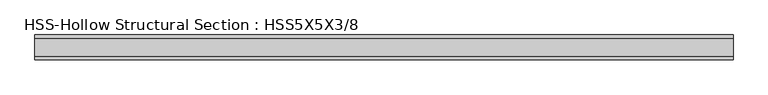
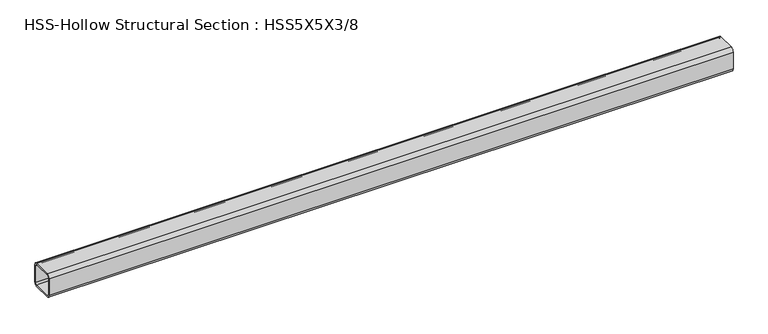
"""IFC4 building model written with IfcOpenShell, lengths in millimetres: member geometry, HSS-Hollow Structural Section : HSS5X5X3/8."""

from ifc_helpers import new_model, si_unit, point, frame, frame_2d, origin, place, context, project, spatial, polyline, circle_curve, trimmed, segment, composite_curve, outline, extrude, source, transform, mapped, element, save


def hss_hollow_structural_section_hss5x5x3_8_98c1edb9(model_context):
    return source(origin(), model_context, "Body", "SweptSolid", [
        extrude(outline(composite_curve([segment(polyline([(63.5, 45.7708), (63.5, -45.7708)]), True, "CONTINUOUS"), segment(trimmed(circle_curve(frame_2d((45.7708, -45.7708)), 17.7292), [point((63.5, -45.7708))], [point((45.7708, -63.5))], False, "CARTESIAN"), True, "CONTINUOUS"), segment(polyline([(45.7708, -63.5), (-45.7708, -63.5)]), True, "CONTINUOUS"), segment(trimmed(circle_curve(frame_2d((-45.7708, -45.7708)), 17.7292), [point((-45.7708, -63.5))], [point((-63.5, -45.7708))], False, "CARTESIAN"), True, "CONTINUOUS"), segment(polyline([(-63.5, -45.7708), (-63.5, 45.7708)]), True, "CONTINUOUS"), segment(trimmed(circle_curve(frame_2d((-45.7708, 45.7708)), 17.7292), [point((-63.5, 45.7708))], [point((-45.7708, 63.5))], False, "CARTESIAN"), True, "CONTINUOUS"), segment(polyline([(-45.7708, 63.5), (45.7708, 63.5)]), True, "CONTINUOUS"), segment(trimmed(circle_curve(frame_2d((45.7708, 45.7708)), 17.7292), [point((45.7708, 63.5))], [point((63.5, 45.7708))], False, "CARTESIAN"), True, "CONTINUOUS")], self_intersect=False), holes=[composite_curve([segment(trimmed(circle_curve(frame_2d((-45.7708, 45.7708)), 8.8646), [point((-45.7708, 54.6354))], [point((-54.6354, 45.7708))], True, "CARTESIAN"), True, "CONTINUOUS"), segment(polyline([(-54.6354, 45.7708), (-54.6354, -45.7708)]), True, "CONTINUOUS"), segment(trimmed(circle_curve(frame_2d((-45.7708, -45.7708)), 8.8646), [point((-54.6354, -45.7708))], [point((-45.7708, -54.6354))], True, "CARTESIAN"), True, "CONTINUOUS"), segment(polyline([(-45.7708, -54.6354), (45.7708, -54.6354)]), True, "CONTINUOUS"), segment(trimmed(circle_curve(frame_2d((45.7708, -45.7708)), 8.8646), [point((45.7708, -54.6354))], [point((54.6354, -45.7708))], True, "CARTESIAN"), True, "CONTINUOUS"), segment(polyline([(54.6354, -45.7708), (54.6354, 45.7708)]), True, "CONTINUOUS"), segment(trimmed(circle_curve(frame_2d((45.7708, 45.7708)), 8.8646), [point((54.6354, 45.7708))], [point((45.7708, 54.6354))], True, "CARTESIAN"), True, "CONTINUOUS"), segment(polyline([(45.7708, 54.6354), (-45.7708, 54.6354)]), True, "CONTINUOUS")], self_intersect=False)]), frame((-1774.2408481, 0.0, 0.0), z_axis=(1.0, 0.0, 0.0), x_axis=(0.0, 1.0, 0.0)), (0.0, 0.0, 1.0), 3548.4816962),
    ])


if __name__ == "__main__":
    model = new_model("IFC4")
    model_context = context("Model", 3, world=origin())
    ifc_project = project(units=[si_unit("LENGTHUNIT", "METRE", prefix="MILLI")], contexts=[model_context])
    site = spatial("IfcSite", under=ifc_project)
    building = spatial("IfcBuilding", under=site)
    placement = place(None, origin())
    hss_hollow_structural_section_hss5x5x3_8_shape = hss_hollow_structural_section_hss5x5x3_8_98c1edb9(model_context)
    element("IfcMember", 1, ObjectType="HSS-Hollow Structural Section : HSS5X5X3/8", at=placement, inside=building, context=model_context, shape_type="MappedRepresentation", body=[
        mapped(hss_hollow_structural_section_hss5x5x3_8_shape, transform((0.0, 0.0, 0.0), x_axis=(1.0, 0.0, 0.0), y_axis=(0.0, 1.0, 0.0), z_axis=(0.0, 0.0, 1.0))),
    ])
    save(model, "model.ifc")

# Revit data of these elements
# Type "HSS-Hollow Structural Section : HSS5X5X3/8"
#   Assembly Code = "B10"
#   Shape = "Square"
#   W = 22.3
#   Ht = 0' - 5"
#   Length [instance default] = 5' - 0"
#   b = 0' - 5"
#   kr = 0' - 0.698"
#   t = 0' - 0.349"
#   A = 0.0429167 SF
#   Structural Material [instance default] = Steel ASTM A500, Grade B, Rectangular and Square
# Element 1 (IfcMember, "HSS-Hollow Structural Section : HSS5X5X3/8")
#   Materials on its faces: "Steel ASTM A500, Grade B, Rectangular and Square"
# Materials
#   "Steel ASTM A500, Grade B, Rectangular and Square": class "Metal", colour RGB 199 199 199, transparency 0, Description = "Carbon steel", Cost = 0
